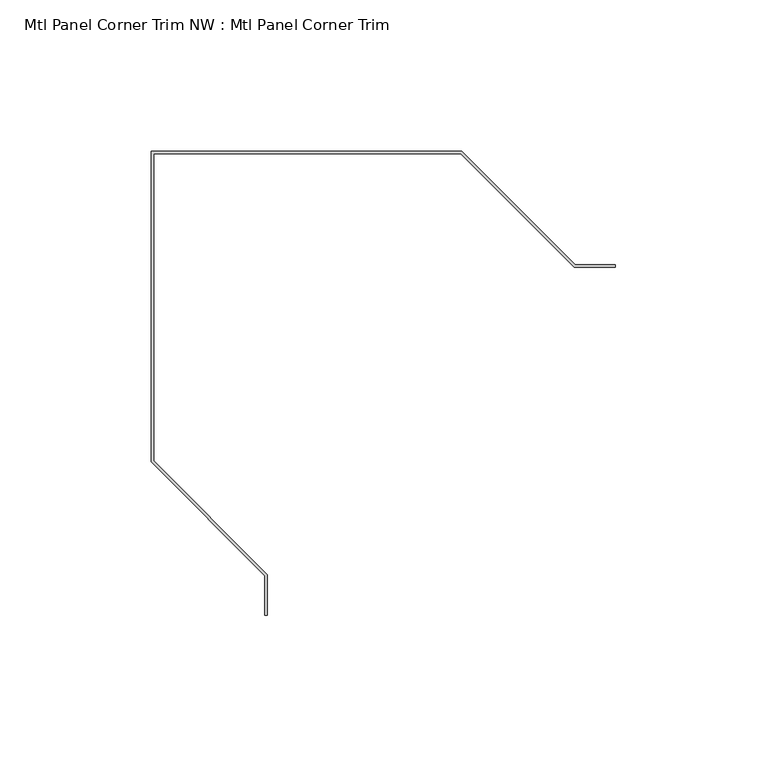
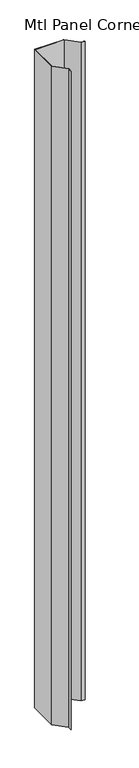
"""IFC4 building model written with IfcOpenShell, lengths in millimetres: proxy geometry, Mtl Panel Corner Trim NW : Mtl Panel Corner Trim."""

import ifcopenshell
import ifcopenshell.guid

model = None  # the IFC model being written
_history = None  # IfcOwnerHistory: only IFC2X3 demands one
_inside = {}  # id of a spatial element -> (the spatial element, [elements in it])
_under = {}  # id of a project, library or spatial element -> (it, [spatial elements below it])
_declared = {}  # id of a project -> (the project, [libraries it declares])
_typed = {}  # id of a type object -> (the type object, [elements of that type])
_made_of = {}  # id of a material, layer set ... -> (it, [elements and type objects made of it])


def new_model(schema):
    """Start an empty IFC model of exactly this schema.

    Asked for "IFC4X3", IfcOpenShell would pick the latest addendum, in which some entities
    have other attributes; the version numbers below select the first issue.
    IFC2X3 requires an IfcOwnerHistory on every rooted entity: one is made here for all.
    """
    global model, _history
    if schema == "IFC4X3":
        model = ifcopenshell.file(schema_version=(4, 3, 0, 0))
    else:
        model = ifcopenshell.file(schema=schema)
    _inside.clear()
    _under.clear()
    _declared.clear()
    _typed.clear()
    _made_of.clear()
    _history = None
    if model.schema == "IFC2X3":
        org = make("IfcOrganization", Name="unknown")
        user = make(
            "IfcPersonAndOrganization",
            ThePerson=make("IfcPerson", FamilyName="unknown"),
            TheOrganization=org,
        )
        app = make(
            "IfcApplication",
            ApplicationDeveloper=org,
            Version="unknown",
            ApplicationFullName="unknown",
            ApplicationIdentifier="unknown",
        )
        _history = make(
            "IfcOwnerHistory",
            OwningUser=user,
            OwningApplication=app,
            ChangeAction="ADDED",
            CreationDate=0,
        )
    return model


def make(cls, **values):
    """One entity of the class cls with the attributes given. An attribute that is None is left unset."""
    return model.create_entity(
        cls, **{name: value for name, value in values.items() if value is not None}
    )


def rooted(cls, **values):
    """An entity with a GlobalId (a new one), such as an element, a storey or a relation."""
    return make(cls, GlobalId=ifcopenshell.guid.new(), OwnerHistory=_history, **values)


def si_unit(unit_type, name, prefix=None):
    """IfcSIUnit, for example si_unit("LENGTHUNIT", "METRE", prefix="MILLI")."""
    return make("IfcSIUnit", UnitType=unit_type, Prefix=prefix, Name=name)


def assignment(units):
    """IfcUnitAssignment: the units of a project."""
    return None if units is None else make("IfcUnitAssignment", Units=units)


def point(xyz):
    """IfcCartesianPoint."""
    return None if xyz is None else make("IfcCartesianPoint", Coordinates=xyz)


def direction(xyz):
    """IfcDirection."""
    return None if xyz is None else make("IfcDirection", DirectionRatios=xyz)


def frame(location, z_axis=None, x_axis=None):
    """IfcAxis2Placement3D, a coordinate frame: its origin and axes. An axis left out is left unset."""
    return make(
        "IfcAxis2Placement3D",
        Location=point(location),
        Axis=direction(z_axis),
        RefDirection=direction(x_axis),
    )


def origin():
    """The frame at (0, 0, 0) with its axes left unset."""
    return frame((0.0, 0.0, 0.0))


def place(relative_to, where):
    """IfcLocalPlacement: puts the frame where relative to a parent placement (None: the world)."""
    return make(
        "IfcLocalPlacement", PlacementRelTo=relative_to, RelativePlacement=where
    )


def context(
    kind, dimensions, precision=None, world=None, true_north=None, identifier=None
):
    """IfcGeometricRepresentationContext, for example the 3D "Model" context."""
    return make(
        "IfcGeometricRepresentationContext",
        ContextIdentifier=identifier,
        ContextType=kind,
        CoordinateSpaceDimension=dimensions,
        Precision=precision,
        WorldCoordinateSystem=world,
        TrueNorth=true_north,
    )


def project(units=None, contexts=None):
    """IfcProject with its units and contexts."""
    return rooted(
        "IfcProject",
        Name="project",
        RepresentationContexts=contexts,
        UnitsInContext=assignment(units),
    )


def spatial(cls, under=None, at=None, **own):
    """A site, building, storey or space (cls), placed at a placement, below another one or the project."""
    s = rooted(cls, ObjectPlacement=at, **own)
    if under is not None:
        _under.setdefault(under.id(), (under, []))[1].append(s)
    return s


def polyline(points):
    """IfcPolyline through the points."""
    return make("IfcPolyline", Points=[point(p) for p in points])


def outline(outer, holes=None, kind="AREA"):
    """IfcArbitraryClosedProfileDef: a profile drawn as a closed curve; with holes, ...WithVoids."""
    if holes is None:
        return make("IfcArbitraryClosedProfileDef", ProfileType=kind, OuterCurve=outer)
    return make(
        "IfcArbitraryProfileDefWithVoids",
        ProfileType=kind,
        OuterCurve=outer,
        InnerCurves=holes,
    )


def extrude(swept, where, along, depth):
    """IfcExtrudedAreaSolid: the profile swept, set in the frame where, extruded along a direction by depth."""
    return make(
        "IfcExtrudedAreaSolid",
        SweptArea=swept,
        Position=where,
        ExtrudedDirection=direction(along),
        Depth=depth,
    )


def shape(context_of_items, identifier, shape_type, items):
    """IfcShapeRepresentation: the items that make up one representation, for example the "Body"."""
    return make(
        "IfcShapeRepresentation",
        ContextOfItems=context_of_items,
        RepresentationIdentifier=identifier,
        RepresentationType=shape_type,
        Items=items,
    )


def source(mapping_origin, context_of_items, identifier, shape_type, items):
    """IfcRepresentationMap: a shape defined once, which mapped items show again and again."""
    return make(
        "IfcRepresentationMap",
        MappingOrigin=mapping_origin,
        MappedRepresentation=shape(context_of_items, identifier, shape_type, items),
    )


def transform(
    local_origin,
    x_axis=None,
    y_axis=None,
    z_axis=None,
    scale=None,
    scale2=None,
    scale3=None,
    uniform=True,
):
    """IfcCartesianTransformationOperator3D, or its non-uniform kind. x_axis, y_axis, z_axis: its Axis1, 2, 3."""
    if uniform:
        return make(
            "IfcCartesianTransformationOperator3D",
            Axis1=direction(x_axis),
            Axis2=direction(y_axis),
            LocalOrigin=point(local_origin),
            Scale=scale,
            Axis3=direction(z_axis),
        )
    return make(
        "IfcCartesianTransformationOperator3DnonUniform",
        Axis1=direction(x_axis),
        Axis2=direction(y_axis),
        LocalOrigin=point(local_origin),
        Scale=scale,
        Axis3=direction(z_axis),
        Scale2=scale2,
        Scale3=scale3,
    )


def mapped(mapping_source, mapping_target):
    """IfcMappedItem: shows the shape of a source again, moved by a transform."""
    return make(
        "IfcMappedItem", MappingSource=mapping_source, MappingTarget=mapping_target
    )


def made_of(thing, what):
    """Note that an element or type object is made of a material, layer set ...; save() writes the relation."""
    if what is not None:
        _made_of.setdefault(what.id(), (what, []))[1].append(thing)
    return thing


def element(
    cls,
    number,
    at=None,
    inside=None,
    cuts=None,
    type_object=None,
    material=None,
    context=None,
    identifier="Body",
    shape_type=None,
    held_by="IfcProductDefinitionShape",
    body=None,
    shapes=None,
    **own,
):
    """One element of the class cls, such as IfcWall. Its Tag is "e" and its number.

    at: its placement. inside: the storey or other place that contains it. cuts: it is an
    opening in that element (IfcRelVoidsElement). A single representation is given by context,
    identifier, shape_type and body (its items); several are given by shapes. held_by: the class
    of the entity that holds the representations. save() writes the other relations.
    """
    e = rooted(cls, Tag="e%d" % number, ObjectPlacement=at, **own)
    if body is not None:
        shapes = [shape(context, identifier, shape_type, body)]
    if shapes is not None:
        e.Representation = make(held_by, Representations=shapes)
    if inside is not None:
        _inside.setdefault(inside.id(), (inside, []))[1].append(e)
    if cuts is not None:
        rooted(
            "IfcRelVoidsElement", RelatingBuildingElement=cuts, RelatedOpeningElement=e
        )
    if type_object is not None:
        _typed.setdefault(type_object.id(), (type_object, []))[1].append(e)
    return made_of(e, material)


def aggregate(whole, parts):
    """IfcRelAggregates: a whole, such as a stair, and the parts it consists of."""
    return rooted("IfcRelAggregates", RelatingObject=whole, RelatedObjects=parts)


def save(model, path):
    """Write the relations noted so far, then the file.

    IfcRelAggregates (storeys below a building ...), IfcRelContainedInSpatialStructure (elements
    in a storey), IfcRelDefinesByType, IfcRelAssociatesMaterial and IfcRelDeclares: one each for
    every whole, place, type object, material and project.
    """
    for whole, parts in _under.values():
        aggregate(whole, parts)
    for where, things in _inside.values():
        rooted(
            "IfcRelContainedInSpatialStructure",
            RelatedElements=things,
            RelatingStructure=where,
        )
    for kind, things in _typed.values():
        rooted("IfcRelDefinesByType", RelatedObjects=things, RelatingType=kind)
    for what, things in _made_of.values():
        rooted("IfcRelAssociatesMaterial", RelatedObjects=things, RelatingMaterial=what)
    for by, libraries in _declared.values():
        rooted("IfcRelDeclares", RelatingContext=by, RelatedDefinitions=libraries)
    model.write(path)


def mtl_panel_corner_trim_nw_mtl_panel_corner_trim_15613486(model_context):
    return source(origin(), model_context, "Body", "SweptSolid", [
        extrude(outline(polyline([(587365.3854739, -531753.7703841), (587364.5980739, -531753.7703841), (587364.5980739, -531740.6345358), (587327.0060739, -531703.0425358), (587327.0060739, -531600.3289841), (587429.7196257, -531600.3289841), (587467.2100257, -531637.8193841), (587480.4474739, -531637.8193841), (587480.4474739, -531638.6131341), (587466.8812437, -531638.6131341), (587429.3908437, -531601.1227341), (587327.7998239, -531601.1227341), (587327.7998239, -531702.7137538), (587365.3854739, -531740.2994038), (587365.3854739, -531753.7703841)])), frame((0.0, 0.0, 6.35), z_axis=(0.0, 0.0, 1.0), x_axis=(1.0, 0.0, 0.0)), (0.0, 0.0, 1.0), 2432.05),
    ])


if __name__ == "__main__":
    model = new_model("IFC4")
    model_context = context("Model", 3, world=origin())
    ifc_project = project(units=[si_unit("LENGTHUNIT", "METRE", prefix="MILLI")], contexts=[model_context])
    site = spatial("IfcSite", under=ifc_project)
    building = spatial("IfcBuilding", under=site)
    placement = place(None, origin())
    mtl_panel_corner_trim_nw_mtl_panel_corner_trim_shape = mtl_panel_corner_trim_nw_mtl_panel_corner_trim_15613486(model_context)
    element("IfcBuildingElementProxy", 1, Name="Mtl Panel Corner Trim NW : Mtl Panel Corner Trim", ObjectType="Mtl Panel Corner Trim NW : Mtl Panel Corner Trim", at=placement, inside=building, context=model_context, shape_type="MappedRepresentation", body=[
        mapped(mtl_panel_corner_trim_nw_mtl_panel_corner_trim_shape, transform((0.0, 0.0, 0.0), x_axis=(1.0, 0.0, 0.0), y_axis=(0.0, 1.0, 0.0), z_axis=(0.0, 0.0, 1.0))),
    ])
    save(model, "model.ifc")

# Revit data of these elements
# Element 1 (IfcBuildingElementProxy, "Mtl Panel Corner Trim NW : Mtl Panel Corner Trim")
#   Materials on its faces: "CORNER TRIM BY MTL PANEL MFR."
# Materials
#   "CORNER TRIM BY MTL PANEL MFR.": class "Generic", colour RGB 239 242 240, transparency 0, Cost = 0
